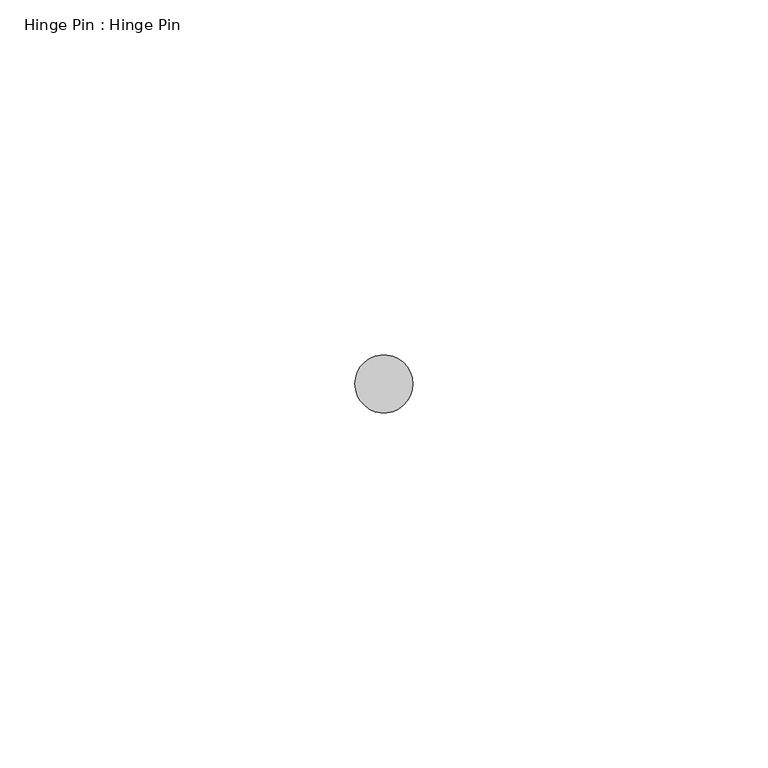
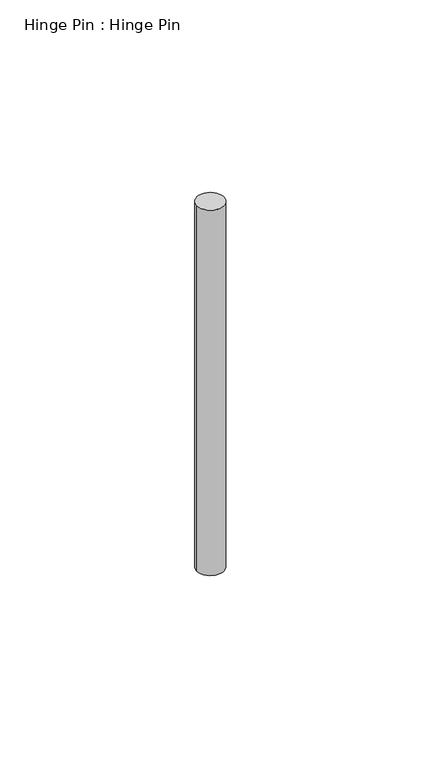
"""IFC4 building model written with IfcOpenShell, lengths in millimetres: proxy geometry, Hinge Pin : Hinge Pin."""

from ifc_helpers import new_model, si_unit, point, frame, frame_2d, origin, place, context, project, spatial, circle_curve, trimmed, segment, composite_curve, outline, extrude, source, transform, mapped, element, save


def hinge_pin_hinge_pin_59ca42a9(model_context):
    return source(origin(), model_context, "Body", "SweptSolid", [
        extrude(outline(composite_curve([segment(trimmed(circle_curve(frame_2d((587319.1320739, -531776.6049841)), 4.0894), [point((587315.0426739, -531776.6049841))], [point((587323.2214739, -531776.6049841))], False, "CARTESIAN"), True, "CONTINUOUS"), segment(trimmed(circle_curve(frame_2d((587319.1320739, -531776.6049841)), 4.0894), [point((587323.2214739, -531776.6049841))], [point((587315.0426739, -531776.6049841))], False, "CARTESIAN"), True, "CONTINUOUS")], self_intersect=False)), frame((0.0, 0.0, 315.7140625), z_axis=(0.0, 0.0, 1.0), x_axis=(1.0, 0.0, 0.0)), (0.0, 0.0, 1.0), 117.871875),
    ])


if __name__ == "__main__":
    model = new_model("IFC4")
    model_context = context("Model", 3, world=origin())
    ifc_project = project(units=[si_unit("LENGTHUNIT", "METRE", prefix="MILLI")], contexts=[model_context])
    site = spatial("IfcSite", under=ifc_project)
    building = spatial("IfcBuilding", under=site)
    placement = place(None, origin())
    hinge_pin_hinge_pin_shape = hinge_pin_hinge_pin_59ca42a9(model_context)
    element("IfcBuildingElementProxy", 1, Name="Hinge Pin : Hinge Pin", ObjectType="Hinge Pin : Hinge Pin", at=placement, inside=building, context=model_context, shape_type="MappedRepresentation", body=[
        mapped(hinge_pin_hinge_pin_shape, transform((0.0, 0.0, 0.0), x_axis=(1.0, 0.0, 0.0), y_axis=(0.0, 1.0, 0.0), z_axis=(0.0, 0.0, 1.0))),
    ])
    save(model, "model.ifc")

# Revit data of these elements
# Element 1 (IfcBuildingElementProxy, "Hinge Pin : Hinge Pin")
#   Materials on its faces: "6\"X6\" WELD-ON STL BUTT HINGE"
# Materials
#   "6\"X6\" WELD-ON STL BUTT HINGE": class "Metal", colour RGB 189 187 185, transparency 0, Description = "Carbon steel", Cost = 0
